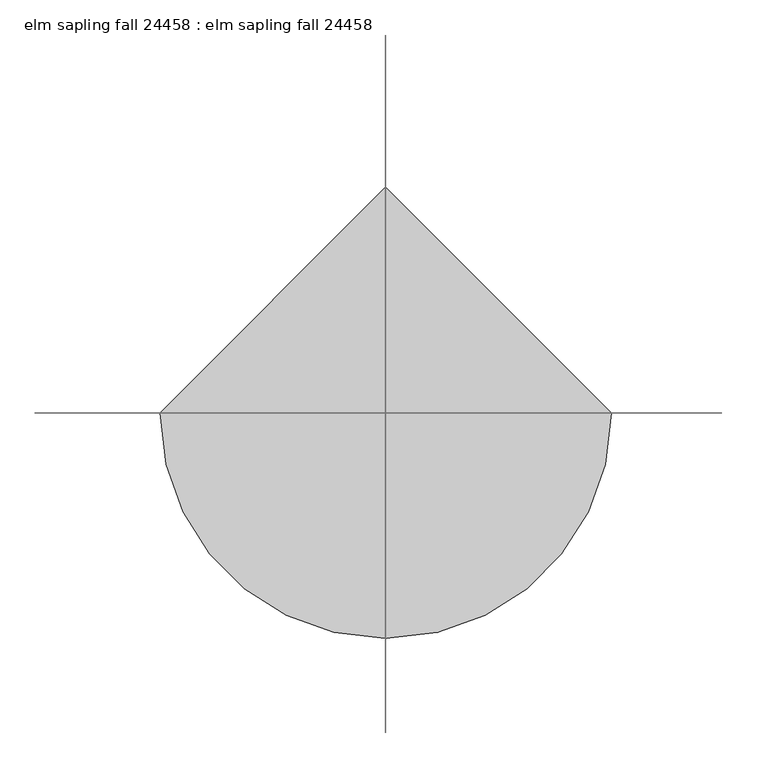
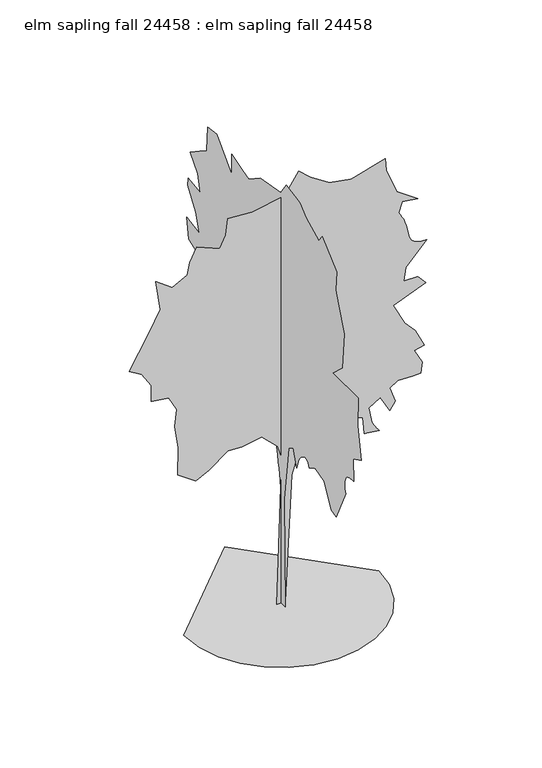
"""IFC4 building model written with IfcOpenShell, lengths in millimetres: proxy geometry, elm sapling fall 24458 : elm sapling fall 24458."""

import ifcopenshell
import ifcopenshell.guid

model = None  # the IFC model being written
_history = None  # IfcOwnerHistory: only IFC2X3 demands one
_inside = {}  # id of a spatial element -> (the spatial element, [elements in it])
_under = {}  # id of a project, library or spatial element -> (it, [spatial elements below it])
_declared = {}  # id of a project -> (the project, [libraries it declares])
_typed = {}  # id of a type object -> (the type object, [elements of that type])
_made_of = {}  # id of a material, layer set ... -> (it, [elements and type objects made of it])


def new_model(schema):
    """Start an empty IFC model of exactly this schema.

    Asked for "IFC4X3", IfcOpenShell would pick the latest addendum, in which some entities
    have other attributes; the version numbers below select the first issue.
    IFC2X3 requires an IfcOwnerHistory on every rooted entity: one is made here for all.
    """
    global model, _history
    if schema == "IFC4X3":
        model = ifcopenshell.file(schema_version=(4, 3, 0, 0))
    else:
        model = ifcopenshell.file(schema=schema)
    _inside.clear()
    _under.clear()
    _declared.clear()
    _typed.clear()
    _made_of.clear()
    _history = None
    if model.schema == "IFC2X3":
        org = make("IfcOrganization", Name="unknown")
        user = make(
            "IfcPersonAndOrganization",
            ThePerson=make("IfcPerson", FamilyName="unknown"),
            TheOrganization=org,
        )
        app = make(
            "IfcApplication",
            ApplicationDeveloper=org,
            Version="unknown",
            ApplicationFullName="unknown",
            ApplicationIdentifier="unknown",
        )
        _history = make(
            "IfcOwnerHistory",
            OwningUser=user,
            OwningApplication=app,
            ChangeAction="ADDED",
            CreationDate=0,
        )
    return model


def make(cls, **values):
    """One entity of the class cls with the attributes given. An attribute that is None is left unset."""
    return model.create_entity(
        cls, **{name: value for name, value in values.items() if value is not None}
    )


def rooted(cls, **values):
    """An entity with a GlobalId (a new one), such as an element, a storey or a relation."""
    return make(cls, GlobalId=ifcopenshell.guid.new(), OwnerHistory=_history, **values)


def si_unit(unit_type, name, prefix=None):
    """IfcSIUnit, for example si_unit("LENGTHUNIT", "METRE", prefix="MILLI")."""
    return make("IfcSIUnit", UnitType=unit_type, Prefix=prefix, Name=name)


def assignment(units):
    """IfcUnitAssignment: the units of a project."""
    return None if units is None else make("IfcUnitAssignment", Units=units)


def point(xyz):
    """IfcCartesianPoint."""
    return None if xyz is None else make("IfcCartesianPoint", Coordinates=xyz)


def direction(xyz):
    """IfcDirection."""
    return None if xyz is None else make("IfcDirection", DirectionRatios=xyz)


def frame(location, z_axis=None, x_axis=None):
    """IfcAxis2Placement3D, a coordinate frame: its origin and axes. An axis left out is left unset."""
    return make(
        "IfcAxis2Placement3D",
        Location=point(location),
        Axis=direction(z_axis),
        RefDirection=direction(x_axis),
    )


def origin():
    """The frame at (0, 0, 0) with its axes left unset."""
    return frame((0.0, 0.0, 0.0))


def place(relative_to, where):
    """IfcLocalPlacement: puts the frame where relative to a parent placement (None: the world)."""
    return make(
        "IfcLocalPlacement", PlacementRelTo=relative_to, RelativePlacement=where
    )


def context(
    kind, dimensions, precision=None, world=None, true_north=None, identifier=None
):
    """IfcGeometricRepresentationContext, for example the 3D "Model" context."""
    return make(
        "IfcGeometricRepresentationContext",
        ContextIdentifier=identifier,
        ContextType=kind,
        CoordinateSpaceDimension=dimensions,
        Precision=precision,
        WorldCoordinateSystem=world,
        TrueNorth=true_north,
    )


def project(units=None, contexts=None):
    """IfcProject with its units and contexts."""
    return rooted(
        "IfcProject",
        Name="project",
        RepresentationContexts=contexts,
        UnitsInContext=assignment(units),
    )


def spatial(cls, under=None, at=None, **own):
    """A site, building, storey or space (cls), placed at a placement, below another one or the project."""
    s = rooted(cls, ObjectPlacement=at, **own)
    if under is not None:
        _under.setdefault(under.id(), (under, []))[1].append(s)
    return s


def point_list(points):
    """IfcCartesianPointList2D or 3D."""
    cls = (
        "IfcCartesianPointList2D" if len(points[0]) == 2 else "IfcCartesianPointList3D"
    )
    return make(cls, CoordList=points)


def triangles(points, corners, closed=None, point_numbers=None):
    """IfcTriangulatedFaceSet: each triangle names its three corners, points numbered from 1."""
    return make(
        "IfcTriangulatedFaceSet",
        Coordinates=point_list(points),
        Closed=closed,
        CoordIndex=corners,
        PnIndex=point_numbers,
    )


def shape(context_of_items, identifier, shape_type, items):
    """IfcShapeRepresentation: the items that make up one representation, for example the "Body"."""
    return make(
        "IfcShapeRepresentation",
        ContextOfItems=context_of_items,
        RepresentationIdentifier=identifier,
        RepresentationType=shape_type,
        Items=items,
    )


def source(mapping_origin, context_of_items, identifier, shape_type, items):
    """IfcRepresentationMap: a shape defined once, which mapped items show again and again."""
    return make(
        "IfcRepresentationMap",
        MappingOrigin=mapping_origin,
        MappedRepresentation=shape(context_of_items, identifier, shape_type, items),
    )


def transform(
    local_origin,
    x_axis=None,
    y_axis=None,
    z_axis=None,
    scale=None,
    scale2=None,
    scale3=None,
    uniform=True,
):
    """IfcCartesianTransformationOperator3D, or its non-uniform kind. x_axis, y_axis, z_axis: its Axis1, 2, 3."""
    if uniform:
        return make(
            "IfcCartesianTransformationOperator3D",
            Axis1=direction(x_axis),
            Axis2=direction(y_axis),
            LocalOrigin=point(local_origin),
            Scale=scale,
            Axis3=direction(z_axis),
        )
    return make(
        "IfcCartesianTransformationOperator3DnonUniform",
        Axis1=direction(x_axis),
        Axis2=direction(y_axis),
        LocalOrigin=point(local_origin),
        Scale=scale,
        Axis3=direction(z_axis),
        Scale2=scale2,
        Scale3=scale3,
    )


def mapped(mapping_source, mapping_target):
    """IfcMappedItem: shows the shape of a source again, moved by a transform."""
    return make(
        "IfcMappedItem", MappingSource=mapping_source, MappingTarget=mapping_target
    )


def made_of(thing, what):
    """Note that an element or type object is made of a material, layer set ...; save() writes the relation."""
    if what is not None:
        _made_of.setdefault(what.id(), (what, []))[1].append(thing)
    return thing


def element(
    cls,
    number,
    at=None,
    inside=None,
    cuts=None,
    type_object=None,
    material=None,
    context=None,
    identifier="Body",
    shape_type=None,
    held_by="IfcProductDefinitionShape",
    body=None,
    shapes=None,
    **own,
):
    """One element of the class cls, such as IfcWall. Its Tag is "e" and its number.

    at: its placement. inside: the storey or other place that contains it. cuts: it is an
    opening in that element (IfcRelVoidsElement). A single representation is given by context,
    identifier, shape_type and body (its items); several are given by shapes. held_by: the class
    of the entity that holds the representations. save() writes the other relations.
    """
    e = rooted(cls, Tag="e%d" % number, ObjectPlacement=at, **own)
    if body is not None:
        shapes = [shape(context, identifier, shape_type, body)]
    if shapes is not None:
        e.Representation = make(held_by, Representations=shapes)
    if inside is not None:
        _inside.setdefault(inside.id(), (inside, []))[1].append(e)
    if cuts is not None:
        rooted(
            "IfcRelVoidsElement", RelatingBuildingElement=cuts, RelatedOpeningElement=e
        )
    if type_object is not None:
        _typed.setdefault(type_object.id(), (type_object, []))[1].append(e)
    return made_of(e, material)


def aggregate(whole, parts):
    """IfcRelAggregates: a whole, such as a stair, and the parts it consists of."""
    return rooted("IfcRelAggregates", RelatingObject=whole, RelatedObjects=parts)


def save(model, path):
    """Write the relations noted so far, then the file.

    IfcRelAggregates (storeys below a building ...), IfcRelContainedInSpatialStructure (elements
    in a storey), IfcRelDefinesByType, IfcRelAssociatesMaterial and IfcRelDeclares: one each for
    every whole, place, type object, material and project.
    """
    for whole, parts in _under.values():
        aggregate(whole, parts)
    for where, things in _inside.values():
        rooted(
            "IfcRelContainedInSpatialStructure",
            RelatedElements=things,
            RelatingStructure=where,
        )
    for kind, things in _typed.values():
        rooted("IfcRelDefinesByType", RelatedObjects=things, RelatingType=kind)
    for what, things in _made_of.values():
        rooted("IfcRelAssociatesMaterial", RelatedObjects=things, RelatingMaterial=what)
    for by, libraries in _declared.values():
        rooted("IfcRelDeclares", RelatingContext=by, RelatedDefinitions=libraries)
    model.write(path)


def elm_sapling_fall_24458_elm_sapling_fall_24458_31049f9d(model_context):
    return source(origin(), model_context, "Body", "Tessellation", [
        triangles([(0.0025148, -47.6280294, 0.2352123), (0.0025387, -35.8607222, 765.0426195), (0.0025449, -88.8133471, 1159.2453747), (0.0025404, -141.765729, 1194.5462723), (0.0025326, -182.9510422, 1076.8757658), (0.0025327, -186.8448634, 1094.5084105), (0.0025328, -191.4077208, 1112.0394625), (0.0025327, -197.3083962, 1129.3648584), (0.0025324, -205.2159077, 1146.3803169), (0.0025318, -215.7998365, 1162.9842453), (0.0025308, -229.7284377, 1179.0751236), (0.0025294, -247.6707291, 1194.5462723), (0.0025278, -266.1283961, 1205.729892), (0.0025263, -281.497934, 1209.8142357), (0.0025249, -294.2944458, 1207.9777925), (0.0025236, -305.0310179, 1201.4093708), (0.0025223, -314.2258055, 1191.2874596), (0.0025211, -322.3919131, 1178.8007944), (0.0025199, -330.0423909, 1165.1280098), (0.0025138, -400.6441861, 1206.314086), (0.0025019, -506.5494587, 1176.8958235), (0.0024887, -588.9190676, 1023.921876), (0.0024827, -641.8729574, 1006.2714272), (0.0024778, -753.6609015, 1235.7324211), (0.0024787, -749.955023, 1252.1128166), (0.0024795, -746.7140144, 1268.4424885), (0.0024803, -744.3975134, 1284.6705677), (0.0024808, -743.4703897, 1300.7435692), (0.0024812, -744.3975134, 1316.61106), (0.0024813, -747.6410654, 1332.2192642), (0.0024812, -753.6609015, 1347.5202198), (0.0024806, -762.4264275, 1360.5910789), (0.0024798, -773.3535221, 1369.9586758), (0.0024786, -786.0814516, 1376.2348915), (0.0024773, -800.2495548, 1380.0423626), (0.0024757, -815.4997141, 1381.9982025), (0.0024741, -831.4686522, 1382.7195248), (0.0024724, -847.798324, 1382.8211174), (0.0024777, -841.9156889, 1541.6803162), (0.0024693, -936.0531115, 1588.7491001), (0.0024803, -894.8670353, 1812.3248428), (0.0024856, -900.7522139, 2012.3675743), (0.0025163, -606.5695527, 2012.3675743), (0.0025083, -712.4748253, 2112.3901028), (0.0025135, -736.0104527, 2371.2693592), (0.002525, -671.2912199, 2530.1260872), (0.0025315, -635.9877789, 2624.2508652), (0.0025343, -647.7555925, 2759.5818489), (0.002556, -483.0163748, 2912.5661156), (0.0025587, -441.8302986, 2859.6071388), (0.0025762, -294.7389499, 2930.2191078), (0.0025861, -218.2529753, 2994.9381226), (0.0026035, -59.3955888, 3024.3514435), (0.0026075, 5.324168, 2930.2191078), (0.0026314, 246.5521201, 2889.0201691), (0.0026429, 381.8761456, 2800.7807877), (0.0026508, 452.4779408, 2818.4337799), (0.0026649, 576.0336622, 2859.6071388), (0.0026605, 576.0336622, 2712.5158264), (0.0026844, 752.5433098, 2894.9131233), (0.0026951, 858.4460026, 2883.1527946), (0.0026932, 864.3311811, 2800.7807877), (0.0026911, 870.2138163, 2706.6228722), (0.0026981, 952.5859686, 2653.6894753), (0.0027074, 1064.37384, 2577.184552), (0.0026953, 976.1190525, 2477.172052), (0.0026887, 946.70079, 2359.5016182), (0.0027039, 1087.9069965, 2377.1519943), (0.002703, 1093.7921751, 2324.2007206), (0.0026891, 999.6546799, 2188.8771492), (0.0026811, 958.4686037, 2065.3214642), (0.0026972, 1105.5599888, 2088.8544754), (0.0026905, 1082.0243614, 1947.6484142), (0.0026803, 993.7695013, 1912.3475166), (0.002667, 870.2138163, 1900.5796303), (0.0026603, 840.7955538, 1777.0239452), (0.0026451, 740.7754961, 1618.1673626), (0.0026388, 681.9388985, 1612.2821114), (0.00263, 611.3345598, 1565.2134727), (0.0026307, 652.520636, 1441.6576424), (0.0026227, 599.5692896, 1359.2881062), (0.00262, 605.4519247, 1247.5001621), (0.0026253, 681.9388985, 1159.2453747), (0.0026163, 605.4519247, 1123.9444771), (0.0026168, 570.1510271, 1265.1506836), (0.0026099, 505.431867, 1259.2654324), (0.002601, 440.7101272, 1188.6636372), (0.0025991, 452.4779408, 1082.7584009), (0.0025979, 470.128426, 982.7383432), (0.0025922, 399.5265944, 1035.6896896), (0.0025979, 411.2944081, 1188.6636372), (0.0025945, 358.3405183, 1259.2654324), (0.0025769, 187.7160856, 1265.1506836), (0.0025618, 70.0440258, 1171.0131884), (0.0025547, 40.7118636, 1033.1496557), (0.0025524, 31.8950213, 989.3575613), (0.0025503, 23.9014662, 947.417098), (0.0025484, 16.9372463, 907.7930632), (0.0025468, 11.2080504, 870.9478558), (0.0025448, 7.7087955, 817.6358482), (0.0025422, 6.9883753, 731.9032179), (0.002539, 8.5836472, 619.1552307), (0.0025228, 28.8589602, 0.2352169), (-30.3527349, -0.0131541, 0.0), (5.2258449, -0.0132761, 1037.8131065), (-24.4228779, -0.0132836, 1126.7587675), (-131.1584368, -0.0132999, 1233.4946217), (-267.5431716, -0.0132894, 1209.7760839), (-362.4197388, -0.0132959, 1215.7045012), (-486.9432063, -0.0132786, 1120.830423), (-575.8889036, -0.0132799, 1073.3908768), (-700.4148783, -0.0132933, 1162.3365377), (-694.4839903, -0.0133135, 1352.0897083), (-718.2049988, -0.0133287, 1512.1934532), (-706.3432228, -0.0133418, 1630.7885399), (-759.7111862, -0.0133608, 1731.5935787), (-878.3062729, -0.0133555, 1749.3836266), (-878.3062729, -0.0133673, 1862.0478252), (-943.5333961, -0.0133855, 1962.8528641), (-1026.5507853, -0.0133861, 2016.2206821), (-896.0963934, -0.0134174, 2241.5516956), (-819.0099649, -0.0134368, 2383.8652473), (-848.6593906, -0.0134573, 2597.3266365), (-735.9926485, -0.0134554, 2514.32211), (-635.1876823, -0.0134554, 2567.6848412), (-617.3975618, -0.0134651, 2650.7175636), (-569.9605227, -0.0134778, 2745.5864822), (-415.7876658, -0.0134686, 2680.359359), (-374.2790076, -0.0134798, 2763.3665016), (-362.4197388, -0.0134922, 2876.0407288), (-196.3856146, -0.0134893, 2864.1789528), (23.0151082, -0.0134951, 2905.6825241), (117.8912597, -0.0135156, 3047.9988373), (194.9779425, -0.0135012, 2976.8534706), (325.4322799, -0.0135003, 2893.8207481), (473.6767922, -0.0134945, 2864.1789528), (704.9361139, -0.0135035, 2929.4063667), (710.8670019, -0.0134952, 2846.3989334), (782.0225424, -0.0134693, 2668.497583), (924.3360941, -0.0134557, 2567.6848412), (817.6027834, -0.0134628, 2585.4904404), (793.8817749, -0.013454, 2514.32211), (805.2762102, -0.0134526, 2495.147699), (816.4090336, -0.0134512, 2475.3026894), (827.0236473, -0.0134381, 2454.1063087), (836.8610556, -0.0134362, 2430.8882492), (845.6596464, -0.0134341, 2404.9751507), (853.1628222, -0.0134315, 2375.6890022), (859.1089708, -0.0134283, 2342.3590599), (866.7848104, -0.0134256, 2311.4472839), (879.1291878, -0.0134239, 2288.9379021), (895.3623539, -0.0134233, 2273.4311451), (914.706958, -0.0134234, 2263.525209), (936.3884108, -0.0134241, 2257.8203247), (959.6218037, -0.0134252, 2254.9171589), (983.6349455, -0.0134149, 2253.4108555), (841.3213211, -0.0134025, 2105.1688866), (829.4620886, -0.0133919, 2010.2924103), (924.3386375, -0.013386, 2010.2924103), (977.7040575, -0.013383, 1950.9935589), (758.3040047, -0.0133722, 1862.0478252), (835.3904331, -0.0133492, 1707.8749683), (906.548517, -0.0133454, 1630.7885399), (965.8447523, -0.0133359, 1506.2625652), (900.6176291, -0.0133302, 1488.4749882), (953.9855198, -0.0133112, 1387.6674786), (942.1262873, -0.0133031, 1316.5119381), (888.7583239, -0.0133109, 1310.5810501), (787.9534304, -0.0133055, 1316.5119381), (734.585467, -0.0132986, 1280.9316971), (770.1632372, -0.0132896, 1174.1983864), (734.585467, -0.0132819, 1120.830423), (669.3583437, -0.0133014, 1233.4946217), (592.2718789, -0.0132918, 1186.0576189), (610.0594923, -0.0132836, 1097.1094145), (613.6383436, -0.0132823, 1082.2071991), (619.0840868, -0.0132811, 1067.9273294), (626.086857, -0.0132801, 1054.1681402), (634.3317026, -0.0132792, 1040.8204811), (643.5138456, -0.0132784, 1027.7851576), (653.3156456, -0.013266, 1014.9581789), (663.427383, -0.0132653, 1002.2353363), (562.6224895, -0.0132721, 1014.0945688), (550.7632207, -0.0132838, 1132.6896555), (479.6051368, -0.0132936, 1156.4081932), (408.4496326, -0.0132955, 1215.7045012), (289.8545278, -0.0133007, 1221.6353165), (289.8545278, -0.013273, 1067.4625322), (224.6268414, -0.0132801, 1061.5316442), (242.4159808, -0.0132953, 1197.9168514), (147.5399042, -0.0132841, 1144.5489607), (70.4532214, -0.013253, 889.5685942), (28.944813, -0.0131461, 0.1174198), (-660.3032278, 1.02e-05, 0.2309946), (-642.8483339, -151.2980869, 0.2309847), (-593.1329455, -290.2406053, 0.2309735), (-515.139741, -412.8488917, 0.2309614), (-412.8488917, -515.139741, 0.2309492), (-290.2406053, -593.1329455, 0.2309372), (-151.2978325, -642.8483339, 0.230926), (2.89e-05, -660.3032278, 0.2309159), (151.2980869, -642.8483339, 0.230908), (290.2406053, -593.1329455, 0.2309027), (412.8488917, -515.139741, 0.2309001), (515.139741, -412.8488917, 0.2309001), (593.1329455, -290.2406053, 0.2309027), (642.8483339, -151.2978325, 0.230908), (660.3032278, 5.88e-05, 0.2309159), (-8.66e-05, 660.3032278, 0.2309946)], [[4, 5, 6], [4, 6, 7], [88, 89, 90], [88, 90, 91], [87, 88, 91], [4, 7, 8], [4, 8, 9], [71, 72, 73], [71, 73, 74], [57, 58, 59], [82, 83, 84], [82, 84, 85], [81, 82, 85], [71, 74, 75], [64, 65, 66], [48, 49, 50], [4, 9, 10], [102, 103, 1], [102, 1, 2], [101, 102, 2], [100, 101, 2], [100, 2, 3], [99, 100, 3], [98, 99, 3], [97, 98, 3], [96, 97, 3], [95, 96, 3], [37, 38, 39], [41, 42, 43], [18, 19, 20], [94, 95, 3], [67, 68, 69], [67, 69, 70], [36, 37, 39], [22, 23, 24], [21, 22, 24], [21, 24, 25], [21, 25, 26], [60, 61, 62], [59, 60, 62], [59, 62, 63], [21, 26, 27], [17, 18, 20], [39, 40, 41], [35, 36, 39], [4, 10, 11], [47, 48, 50], [21, 27, 28], [81, 85, 86], [39, 41, 43], [52, 53, 54], [34, 35, 39], [21, 28, 29], [16, 17, 20], [51, 52, 54], [56, 57, 59], [87, 91, 92], [86, 87, 92], [76, 77, 78], [79, 80, 81], [4, 11, 12], [63, 64, 66], [59, 63, 66], [59, 66, 67], [21, 29, 30], [20, 21, 30], [20, 30, 31], [81, 86, 92], [79, 81, 92], [79, 92, 93], [34, 39, 43], [33, 34, 43], [32, 33, 43], [31, 32, 43], [20, 31, 43], [16, 20, 43], [15, 16, 43], [14, 15, 43], [13, 14, 43], [43, 44, 45], [43, 45, 46], [94, 3, 4], [93, 94, 4], [12, 13, 43], [4, 12, 43], [93, 4, 43], [79, 93, 43], [79, 43, 46], [79, 46, 47], [79, 47, 50], [79, 50, 51], [79, 51, 54], [79, 54, 55], [79, 55, 56], [79, 56, 59], [79, 59, 67], [78, 79, 67], [76, 78, 67], [75, 76, 67], [71, 75, 67], [71, 67, 70], [139, 140, 141], [181, 182, 183], [122, 123, 124], [155, 156, 157], [180, 181, 183], [154, 155, 157], [171, 172, 173], [170, 171, 173], [179, 180, 183], [159, 160, 161], [158, 159, 161], [153, 154, 157], [179, 183, 184], [178, 179, 184], [177, 178, 184], [176, 177, 184], [175, 176, 184], [174, 175, 184], [188, 189, 190], [187, 188, 190], [136, 137, 138], [163, 164, 165], [132, 133, 134], [193, 104, 105], [192, 193, 105], [191, 192, 105], [191, 105, 106], [129, 130, 131], [152, 153, 157], [119, 120, 121], [126, 127, 128], [116, 117, 118], [166, 167, 168], [174, 184, 185], [125, 126, 128], [165, 166, 168], [165, 168, 169], [151, 152, 157], [136, 138, 139], [110, 111, 112], [110, 112, 113], [109, 110, 113], [109, 113, 114], [109, 114, 115], [132, 134, 135], [174, 185, 186], [191, 106, 107], [190, 191, 107], [108, 109, 115], [107, 108, 115], [162, 163, 165], [162, 165, 169], [162, 169, 170], [118, 119, 121], [139, 141, 142], [136, 139, 142], [173, 174, 186], [162, 170, 173], [162, 173, 186], [161, 162, 186], [161, 186, 187], [150, 151, 157], [116, 118, 121], [116, 121, 122], [116, 122, 124], [116, 124, 125], [116, 125, 128], [115, 116, 128], [107, 115, 128], [190, 107, 128], [187, 190, 128], [161, 187, 128], [158, 161, 128], [157, 158, 128], [150, 157, 128], [149, 150, 128], [148, 149, 128], [147, 148, 128], [146, 147, 128], [145, 146, 128], [144, 145, 128], [143, 144, 128], [142, 143, 128], [136, 142, 128], [135, 136, 128], [132, 135, 128], [131, 132, 128], [129, 131, 128], [208, 209, 194], [207, 208, 194], [207, 194, 195], [206, 207, 195], [206, 195, 196], [206, 196, 197], [205, 206, 197], [204, 205, 197], [204, 197, 198], [204, 198, 199], [204, 199, 200], [204, 200, 201], [204, 201, 202], [204, 202, 203]], closed=False),
    ])


if __name__ == "__main__":
    model = new_model("IFC4")
    model_context = context("Model", 3, world=origin())
    ifc_project = project(units=[si_unit("LENGTHUNIT", "METRE", prefix="MILLI")], contexts=[model_context])
    site = spatial("IfcSite", under=ifc_project)
    building = spatial("IfcBuilding", under=site)
    placement = place(None, origin())
    elm_sapling_fall_24458_elm_sapling_fall_24458_shape = elm_sapling_fall_24458_elm_sapling_fall_24458_31049f9d(model_context)
    element("IfcBuildingElementProxy", 1, Name="elm sapling fall 24458 : elm sapling fall 24458", ObjectType="elm sapling fall 24458 : elm sapling fall 24458", at=placement, inside=building, context=model_context, shape_type="MappedRepresentation", body=[
        mapped(elm_sapling_fall_24458_elm_sapling_fall_24458_shape, transform((0.0, 0.0, 0.0), x_axis=(1.0, 0.0, 0.0), y_axis=(0.0, 1.0, 0.0), z_axis=(0.0, 0.0, 1.0))),
    ])
    save(model, "model.ifc")

# Revit data of these elements
# Type "elm sapling fall 24458 : elm sapling fall 24458"
#   built-in parameter 1005195 = "RPC-16-FWVN-NVXX-5TD6-C000-ST1L-LVER-AU"
#   Height = 0
